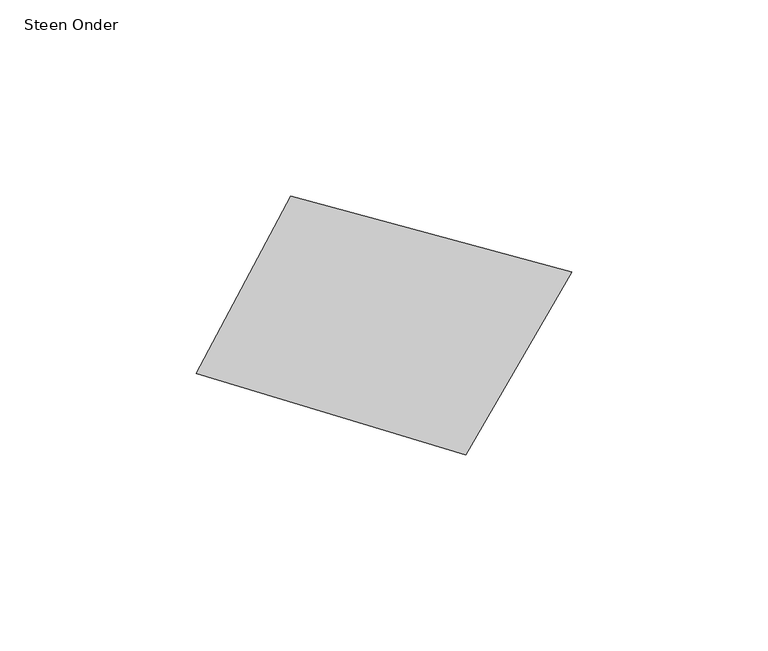
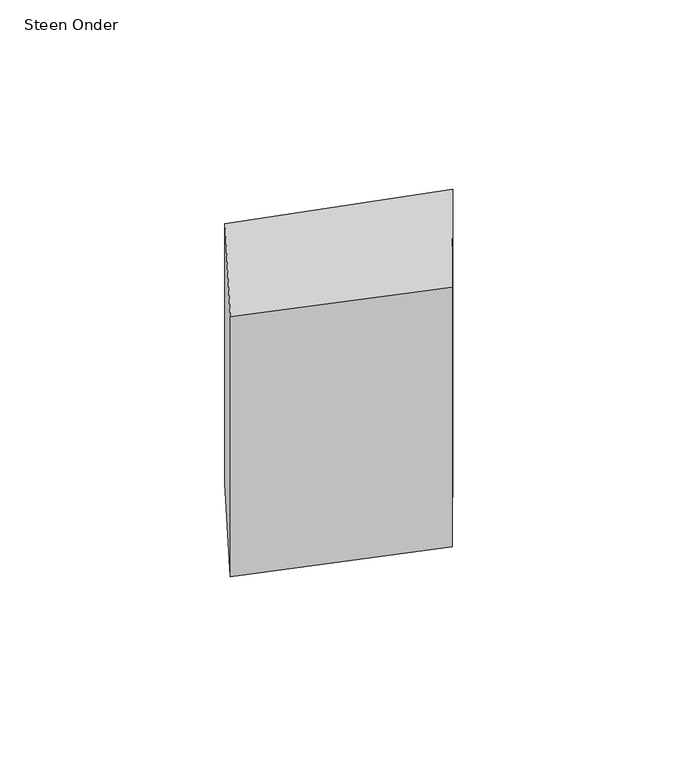
"""IFC4 building model written with IfcOpenShell, lengths in millimetres: proxy geometry, 00_GMA_steen_versie_4 : Steen Onder."""

from ifc_helpers import new_model, si_unit, frame, origin, place, context, project, spatial, polyline, outline, extrude, source, transform, mapped, element, save


def steen_onder_58d5be24(model_context):
    return source(origin(), model_context, "Body", "SweptSolid", [
        extrude(outline(polyline([(136.5603057, 55.1371747), (109.5048572, 8.5579046), (40.7492374, 29.3583534), (64.941042, 74.5887973), (136.5603057, 55.1371747)])), frame((0.0, 0.0, -100.0), z_axis=(0.0, 0.0, 1.0), x_axis=(1.0, 0.0, 0.0)), (0.0, 0.0, 1.0), 100.0),
    ])


if __name__ == "__main__":
    model = new_model("IFC4")
    model_context = context("Model", 3, world=origin())
    ifc_project = project(units=[si_unit("LENGTHUNIT", "METRE", prefix="MILLI")], contexts=[model_context])
    site = spatial("IfcSite", under=ifc_project)
    building = spatial("IfcBuilding", under=site)
    placement = place(None, origin())
    steen_onder_shape = steen_onder_58d5be24(model_context)
    element("IfcBuildingElementProxy", 1, Name="00_GMA_steen_versie_4 : Steen Onder", ObjectType="00_GMA_steen_versie_4 : Steen Onder", at=placement, inside=building, context=model_context, shape_type="MappedRepresentation", body=[
        mapped(steen_onder_shape, transform((0.0, 0.0, 0.0), x_axis=(1.0, 0.0, 0.0), y_axis=(0.0, 1.0, 0.0), z_axis=(0.0, 0.0, 1.0))),
    ])
    save(model, "model.ifc")

# Revit data of these elements
# Type "00_GMA_steen_versie_4 : Steen Onder"
#   StootVoegHalfBoven [instance default] = 5 mm
#   StootVoegHalf [instance default] = 5 mm
#   StootVoegBreedteOnder = 10 mm
#   StootVoegBreedteBoven = 10 mm
#   Steendikte = 100 mm
#   LintVoegOnderHalf = 0 mm
#   LintVoegOnder = 0 mm
#   LintVoegBovenHalf = 5 mm
#   LintVoegBoven = 10 mm
#   materiaal = none
#   MateriaalVoeg = none
#   Default Elevation = 0
